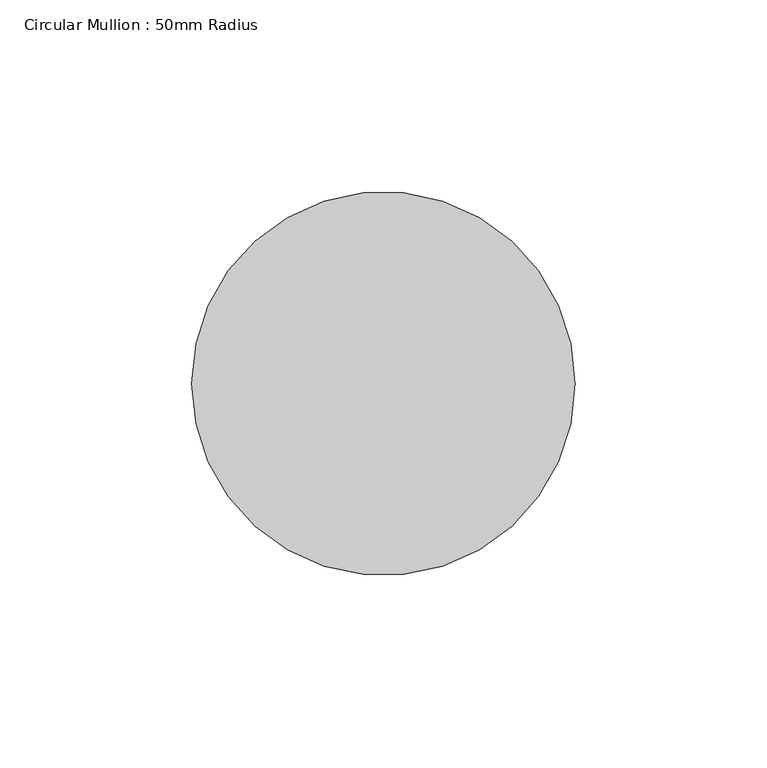
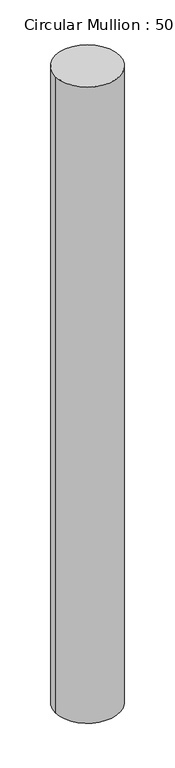
"""IFC4 building model written with IfcOpenShell, lengths in millimetres: member geometry, Circular Mullion : 50mm Radius."""

from ifc_helpers import new_model, si_unit, point, frame, origin, origin_2d, place, context, project, spatial, circle_curve, trimmed, segment, composite_curve, outline, extrude, source, transform, mapped, element, save


def circular_mullion_50mm_radius_04b8ed44(model_context):
    return source(origin(), model_context, "Body", "SweptSolid", [
        extrude(outline(composite_curve([segment(trimmed(circle_curve(origin_2d(), 50.0), [point((50.0, 0.0))], [point((-50.0, 0.0))], False, "CARTESIAN"), True, "CONTINUOUS"), segment(trimmed(circle_curve(origin_2d(), 50.0), [point((-50.0, 0.0))], [point((50.0, 0.0))], False, "CARTESIAN"), True, "CONTINUOUS")], self_intersect=False)), frame((0.0, 0.0, -1050.5460983), z_axis=(0.0, 0.0, 1.0), x_axis=(1.0, 0.0, 0.0)), (0.0, 0.0, 1.0), 1050.5460983),
    ])


if __name__ == "__main__":
    model = new_model("IFC4")
    model_context = context("Model", 3, world=origin())
    ifc_project = project(units=[si_unit("LENGTHUNIT", "METRE", prefix="MILLI")], contexts=[model_context])
    site = spatial("IfcSite", under=ifc_project)
    building = spatial("IfcBuilding", under=site)
    placement = place(None, origin())
    circular_mullion_50mm_radius_shape = circular_mullion_50mm_radius_04b8ed44(model_context)
    element("IfcMember", 1, ObjectType="Circular Mullion : 50mm Radius", at=placement, inside=building, context=model_context, shape_type="MappedRepresentation", body=[
        mapped(circular_mullion_50mm_radius_shape, transform((0.0, 0.0, 0.0), x_axis=(1.0, 0.0, 0.0), y_axis=(0.0, 1.0, 0.0), z_axis=(0.0, 0.0, 1.0))),
    ])
    save(model, "model.ifc")

# Revit data of these elements
# Type "Circular Mullion : 50mm Radius"
#   built-in parameter 1007350 = 0.164042 (stored number, unit not read)
# Element 1 (IfcMember, "Circular Mullion : 50mm Radius")
#   Materials on its faces: "Aluminium"
# Materials
#   "Aluminium": class "Metal", colour RGB 247 247 247, transparency 0, Description = "Aluminium 6061", Cost = 0
